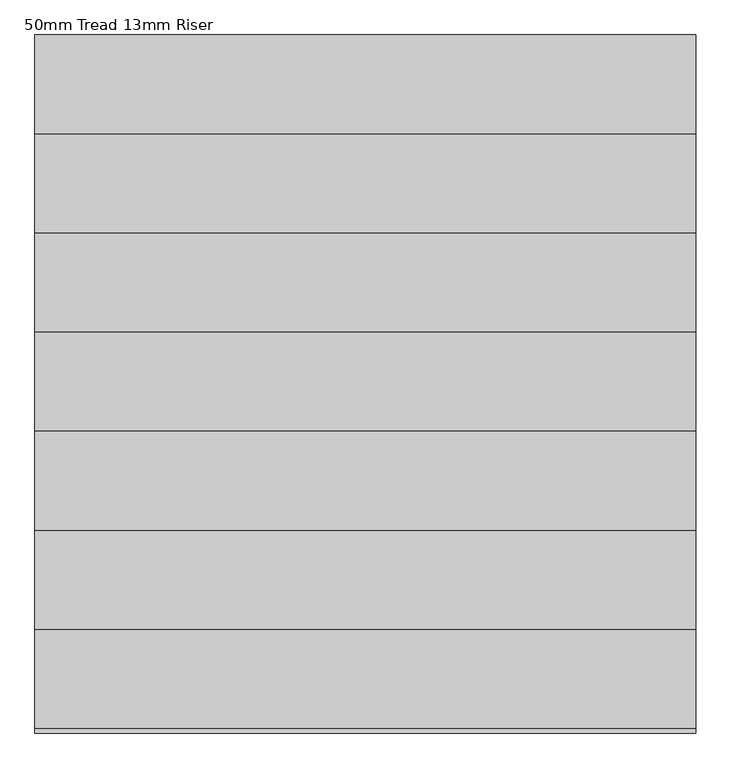
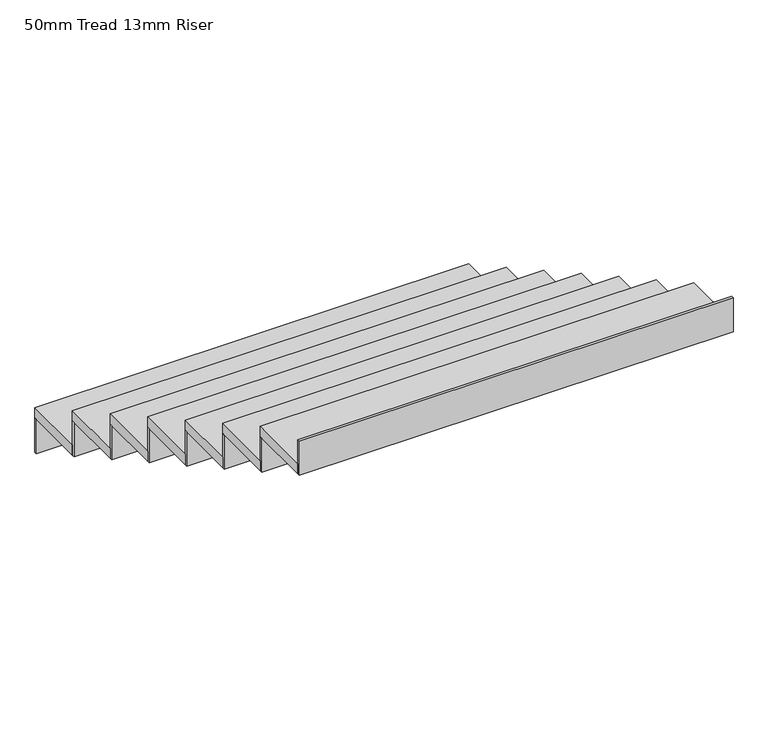
"""IFC4 building model written with IfcOpenShell, lengths in millimetres: stair flight geometry, 50mm Tread 13mm Riser."""

from ifc_helpers import new_model, si_unit, frame, origin, place, context, project, spatial, polyline, outline, extrude, source, transform, mapped, element, save


def stair_flight_50mm_tread_13mm_riser_f31e559f(model_context):
    return source(origin(), model_context, "Body", "SweptSolid", [
        extrude(outline(polyline([(15000.0002442, 23517.4999999), (15000.0002442, 23529.9999999), (17000.0002442, 23529.9999999), (17000.0002442, 23517.4999999), (15000.0002442, 23517.4999999)])), frame((0.0, 0.0, 22283.3333333), z_axis=(0.0, 0.0, 1.0), x_axis=(1.0, 0.0, 0.0)), (0.0, 0.0, 1.0), 166.6666667),
        extrude(outline(polyline([(17000.0002442, 23229.9999999), (15000.0002442, 23229.9999999), (15000.0002442, 23529.9999999), (17000.0002442, 23529.9999999), (17000.0002442, 23229.9999999)])), frame((0.0, 0.0, 22450.0), z_axis=(0.0, 0.0, 1.0), x_axis=(1.0, 0.0, 0.0)), (0.0, 0.0, 1.0), 50.0),
        extrude(outline(polyline([(15000.0002442, 23217.4999999), (15000.0002442, 23229.9999999), (17000.0002442, 23229.9999999), (17000.0002442, 23217.4999999), (15000.0002442, 23217.4999999)])), frame((0.0, 0.0, 22450.0), z_axis=(0.0, 0.0, 1.0), x_axis=(1.0, 0.0, 0.0)), (0.0, 0.0, 1.0), 166.6666667),
        extrude(outline(polyline([(17000.0002442, 22929.9999999), (15000.0002442, 22929.9999999), (15000.0002442, 23229.9999999), (17000.0002442, 23229.9999999), (17000.0002442, 22929.9999999)])), frame((0.0, 0.0, 22616.6666667), z_axis=(0.0, 0.0, 1.0), x_axis=(1.0, 0.0, 0.0)), (0.0, 0.0, 1.0), 50.0),
        extrude(outline(polyline([(15000.0002442, 22917.4999999), (15000.0002442, 22929.9999999), (17000.0002442, 22929.9999999), (17000.0002442, 22917.4999999), (15000.0002442, 22917.4999999)])), frame((0.0, 0.0, 22616.6666667), z_axis=(0.0, 0.0, 1.0), x_axis=(1.0, 0.0, 0.0)), (0.0, 0.0, 1.0), 166.6666667),
        extrude(outline(polyline([(17000.0002442, 22629.9999999), (15000.0002442, 22629.9999999), (15000.0002442, 22929.9999999), (17000.0002442, 22929.9999999), (17000.0002442, 22629.9999999)])), frame((0.0, 0.0, 22783.3333333), z_axis=(0.0, 0.0, 1.0), x_axis=(1.0, 0.0, 0.0)), (0.0, 0.0, 1.0), 50.0),
        extrude(outline(polyline([(15000.0002442, 22617.4999999), (15000.0002442, 22629.9999999), (17000.0002442, 22629.9999999), (17000.0002442, 22617.4999999), (15000.0002442, 22617.4999999)])), frame((0.0, 0.0, 22783.3333333), z_axis=(0.0, 0.0, 1.0), x_axis=(1.0, 0.0, 0.0)), (0.0, 0.0, 1.0), 166.6666667),
        extrude(outline(polyline([(17000.0002442, 22329.9999999), (15000.0002442, 22329.9999999), (15000.0002442, 22629.9999999), (17000.0002442, 22629.9999999), (17000.0002442, 22329.9999999)])), frame((0.0, 0.0, 22950.0), z_axis=(0.0, 0.0, 1.0), x_axis=(1.0, 0.0, 0.0)), (0.0, 0.0, 1.0), 50.0),
        extrude(outline(polyline([(15000.0002442, 22317.4999999), (15000.0002442, 22329.9999999), (17000.0002442, 22329.9999999), (17000.0002442, 22317.4999999), (15000.0002442, 22317.4999999)])), frame((0.0, 0.0, 22950.0), z_axis=(0.0, 0.0, 1.0), x_axis=(1.0, 0.0, 0.0)), (0.0, 0.0, 1.0), 166.6666667),
        extrude(outline(polyline([(17000.0002442, 22029.9999999), (15000.0002442, 22029.9999999), (15000.0002442, 22329.9999999), (17000.0002442, 22329.9999999), (17000.0002442, 22029.9999999)])), frame((0.0, 0.0, 23116.6666667), z_axis=(0.0, 0.0, 1.0), x_axis=(1.0, 0.0, 0.0)), (0.0, 0.0, 1.0), 50.0),
        extrude(outline(polyline([(15000.0002442, 22017.4999999), (15000.0002442, 22029.9999999), (17000.0002442, 22029.9999999), (17000.0002442, 22017.4999999), (15000.0002442, 22017.4999999)])), frame((0.0, 0.0, 23116.6666667), z_axis=(0.0, 0.0, 1.0), x_axis=(1.0, 0.0, 0.0)), (0.0, 0.0, 1.0), 166.6666667),
        extrude(outline(polyline([(17000.0002442, 21729.9999999), (15000.0002442, 21729.9999999), (15000.0002442, 22029.9999999), (17000.0002442, 22029.9999999), (17000.0002442, 21729.9999999)])), frame((0.0, 0.0, 23283.3333333), z_axis=(0.0, 0.0, 1.0), x_axis=(1.0, 0.0, 0.0)), (0.0, 0.0, 1.0), 50.0),
        extrude(outline(polyline([(15000.0002442, 21717.4999999), (15000.0002442, 21729.9999999), (17000.0002442, 21729.9999999), (17000.0002442, 21717.4999999), (15000.0002442, 21717.4999999)])), frame((0.0, 0.0, 23283.3333333), z_axis=(0.0, 0.0, 1.0), x_axis=(1.0, 0.0, 0.0)), (0.0, 0.0, 1.0), 166.6666667),
        extrude(outline(polyline([(15000.0002442, 21417.4999999), (15000.0002442, 21429.9999999), (17000.0002442, 21429.9999999), (17000.0002442, 21417.4999999), (15000.0002442, 21417.4999999)])), frame((0.0, 0.0, 23450.0), z_axis=(0.0, 0.0, 1.0), x_axis=(1.0, 0.0, 0.0)), (0.0, 0.0, 1.0), 166.6666667),
        extrude(outline(polyline([(17000.0002442, 21429.9999999), (15000.0002442, 21429.9999999), (15000.0002442, 21729.9999999), (17000.0002442, 21729.9999999), (17000.0002442, 21429.9999999)])), frame((0.0, 0.0, 23450.0), z_axis=(0.0, 0.0, 1.0), x_axis=(1.0, 0.0, 0.0)), (0.0, 0.0, 1.0), 50.0),
    ])


if __name__ == "__main__":
    model = new_model("IFC4")
    model_context = context("Model", 3, world=origin())
    ifc_project = project(units=[si_unit("LENGTHUNIT", "METRE", prefix="MILLI")], contexts=[model_context])
    site = spatial("IfcSite", under=ifc_project)
    building = spatial("IfcBuilding", under=site)
    placement = place(None, origin())
    stair_flight_50mm_tread_13mm_riser_shape = stair_flight_50mm_tread_13mm_riser_f31e559f(model_context)
    element("IfcStairFlight", 1, ObjectType="50mm Tread 13mm Riser", at=placement, inside=building, context=model_context, shape_type="MappedRepresentation", body=[
        mapped(stair_flight_50mm_tread_13mm_riser_shape, transform((0.0, 0.0, 0.0), x_axis=(1.0, 0.0, 0.0), y_axis=(0.0, 1.0, 0.0), z_axis=(0.0, 0.0, 1.0))),
    ])
    save(model, "model.ifc")
